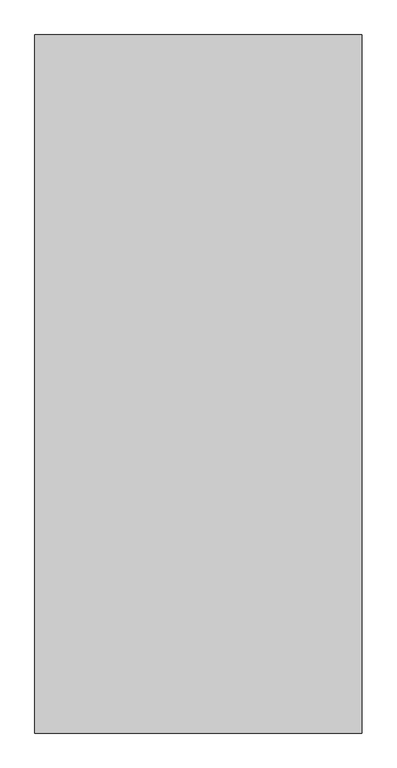
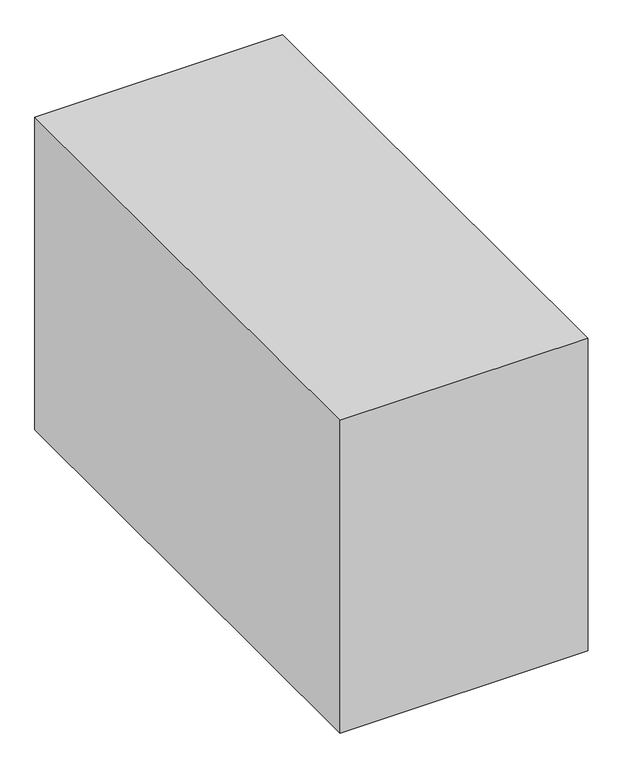
"""IFC4 building model written with IfcOpenShell, lengths in millimetres: proxy geometry, Space Planning Box_hec : Space Planning Box_hec."""

import ifcopenshell
import ifcopenshell.guid

model = None  # the IFC model being written
_history = None  # IfcOwnerHistory: only IFC2X3 demands one
_inside = {}  # id of a spatial element -> (the spatial element, [elements in it])
_under = {}  # id of a project, library or spatial element -> (it, [spatial elements below it])
_declared = {}  # id of a project -> (the project, [libraries it declares])
_typed = {}  # id of a type object -> (the type object, [elements of that type])
_made_of = {}  # id of a material, layer set ... -> (it, [elements and type objects made of it])


def new_model(schema):
    """Start an empty IFC model of exactly this schema.

    Asked for "IFC4X3", IfcOpenShell would pick the latest addendum, in which some entities
    have other attributes; the version numbers below select the first issue.
    IFC2X3 requires an IfcOwnerHistory on every rooted entity: one is made here for all.
    """
    global model, _history
    if schema == "IFC4X3":
        model = ifcopenshell.file(schema_version=(4, 3, 0, 0))
    else:
        model = ifcopenshell.file(schema=schema)
    _inside.clear()
    _under.clear()
    _declared.clear()
    _typed.clear()
    _made_of.clear()
    _history = None
    if model.schema == "IFC2X3":
        org = make("IfcOrganization", Name="unknown")
        user = make(
            "IfcPersonAndOrganization",
            ThePerson=make("IfcPerson", FamilyName="unknown"),
            TheOrganization=org,
        )
        app = make(
            "IfcApplication",
            ApplicationDeveloper=org,
            Version="unknown",
            ApplicationFullName="unknown",
            ApplicationIdentifier="unknown",
        )
        _history = make(
            "IfcOwnerHistory",
            OwningUser=user,
            OwningApplication=app,
            ChangeAction="ADDED",
            CreationDate=0,
        )
    return model


def make(cls, **values):
    """One entity of the class cls with the attributes given. An attribute that is None is left unset."""
    return model.create_entity(
        cls, **{name: value for name, value in values.items() if value is not None}
    )


def rooted(cls, **values):
    """An entity with a GlobalId (a new one), such as an element, a storey or a relation."""
    return make(cls, GlobalId=ifcopenshell.guid.new(), OwnerHistory=_history, **values)


def si_unit(unit_type, name, prefix=None):
    """IfcSIUnit, for example si_unit("LENGTHUNIT", "METRE", prefix="MILLI")."""
    return make("IfcSIUnit", UnitType=unit_type, Prefix=prefix, Name=name)


def assignment(units):
    """IfcUnitAssignment: the units of a project."""
    return None if units is None else make("IfcUnitAssignment", Units=units)


def point(xyz):
    """IfcCartesianPoint."""
    return None if xyz is None else make("IfcCartesianPoint", Coordinates=xyz)


def direction(xyz):
    """IfcDirection."""
    return None if xyz is None else make("IfcDirection", DirectionRatios=xyz)


def frame(location, z_axis=None, x_axis=None):
    """IfcAxis2Placement3D, a coordinate frame: its origin and axes. An axis left out is left unset."""
    return make(
        "IfcAxis2Placement3D",
        Location=point(location),
        Axis=direction(z_axis),
        RefDirection=direction(x_axis),
    )


def origin():
    """The frame at (0, 0, 0) with its axes left unset."""
    return frame((0.0, 0.0, 0.0))


def origin_with_axes():
    """The frame at (0, 0, 0) with the z axis (0, 0, 1) and the x axis (1, 0, 0) written out."""
    return frame((0.0, 0.0, 0.0), z_axis=(0.0, 0.0, 1.0), x_axis=(1.0, 0.0, 0.0))


def place(relative_to, where):
    """IfcLocalPlacement: puts the frame where relative to a parent placement (None: the world)."""
    return make(
        "IfcLocalPlacement", PlacementRelTo=relative_to, RelativePlacement=where
    )


def context(
    kind, dimensions, precision=None, world=None, true_north=None, identifier=None
):
    """IfcGeometricRepresentationContext, for example the 3D "Model" context."""
    return make(
        "IfcGeometricRepresentationContext",
        ContextIdentifier=identifier,
        ContextType=kind,
        CoordinateSpaceDimension=dimensions,
        Precision=precision,
        WorldCoordinateSystem=world,
        TrueNorth=true_north,
    )


def project(units=None, contexts=None):
    """IfcProject with its units and contexts."""
    return rooted(
        "IfcProject",
        Name="project",
        RepresentationContexts=contexts,
        UnitsInContext=assignment(units),
    )


def spatial(cls, under=None, at=None, **own):
    """A site, building, storey or space (cls), placed at a placement, below another one or the project."""
    s = rooted(cls, ObjectPlacement=at, **own)
    if under is not None:
        _under.setdefault(under.id(), (under, []))[1].append(s)
    return s


def polyline(points):
    """IfcPolyline through the points."""
    return make("IfcPolyline", Points=[point(p) for p in points])


def outline(outer, holes=None, kind="AREA"):
    """IfcArbitraryClosedProfileDef: a profile drawn as a closed curve; with holes, ...WithVoids."""
    if holes is None:
        return make("IfcArbitraryClosedProfileDef", ProfileType=kind, OuterCurve=outer)
    return make(
        "IfcArbitraryProfileDefWithVoids",
        ProfileType=kind,
        OuterCurve=outer,
        InnerCurves=holes,
    )


def extrude(swept, where, along, depth):
    """IfcExtrudedAreaSolid: the profile swept, set in the frame where, extruded along a direction by depth."""
    return make(
        "IfcExtrudedAreaSolid",
        SweptArea=swept,
        Position=where,
        ExtrudedDirection=direction(along),
        Depth=depth,
    )


def shape(context_of_items, identifier, shape_type, items):
    """IfcShapeRepresentation: the items that make up one representation, for example the "Body"."""
    return make(
        "IfcShapeRepresentation",
        ContextOfItems=context_of_items,
        RepresentationIdentifier=identifier,
        RepresentationType=shape_type,
        Items=items,
    )


def source(mapping_origin, context_of_items, identifier, shape_type, items):
    """IfcRepresentationMap: a shape defined once, which mapped items show again and again."""
    return make(
        "IfcRepresentationMap",
        MappingOrigin=mapping_origin,
        MappedRepresentation=shape(context_of_items, identifier, shape_type, items),
    )


def transform(
    local_origin,
    x_axis=None,
    y_axis=None,
    z_axis=None,
    scale=None,
    scale2=None,
    scale3=None,
    uniform=True,
):
    """IfcCartesianTransformationOperator3D, or its non-uniform kind. x_axis, y_axis, z_axis: its Axis1, 2, 3."""
    if uniform:
        return make(
            "IfcCartesianTransformationOperator3D",
            Axis1=direction(x_axis),
            Axis2=direction(y_axis),
            LocalOrigin=point(local_origin),
            Scale=scale,
            Axis3=direction(z_axis),
        )
    return make(
        "IfcCartesianTransformationOperator3DnonUniform",
        Axis1=direction(x_axis),
        Axis2=direction(y_axis),
        LocalOrigin=point(local_origin),
        Scale=scale,
        Axis3=direction(z_axis),
        Scale2=scale2,
        Scale3=scale3,
    )


def mapped(mapping_source, mapping_target):
    """IfcMappedItem: shows the shape of a source again, moved by a transform."""
    return make(
        "IfcMappedItem", MappingSource=mapping_source, MappingTarget=mapping_target
    )


def made_of(thing, what):
    """Note that an element or type object is made of a material, layer set ...; save() writes the relation."""
    if what is not None:
        _made_of.setdefault(what.id(), (what, []))[1].append(thing)
    return thing


def element(
    cls,
    number,
    at=None,
    inside=None,
    cuts=None,
    type_object=None,
    material=None,
    context=None,
    identifier="Body",
    shape_type=None,
    held_by="IfcProductDefinitionShape",
    body=None,
    shapes=None,
    **own,
):
    """One element of the class cls, such as IfcWall. Its Tag is "e" and its number.

    at: its placement. inside: the storey or other place that contains it. cuts: it is an
    opening in that element (IfcRelVoidsElement). A single representation is given by context,
    identifier, shape_type and body (its items); several are given by shapes. held_by: the class
    of the entity that holds the representations. save() writes the other relations.
    """
    e = rooted(cls, Tag="e%d" % number, ObjectPlacement=at, **own)
    if body is not None:
        shapes = [shape(context, identifier, shape_type, body)]
    if shapes is not None:
        e.Representation = make(held_by, Representations=shapes)
    if inside is not None:
        _inside.setdefault(inside.id(), (inside, []))[1].append(e)
    if cuts is not None:
        rooted(
            "IfcRelVoidsElement", RelatingBuildingElement=cuts, RelatedOpeningElement=e
        )
    if type_object is not None:
        _typed.setdefault(type_object.id(), (type_object, []))[1].append(e)
    return made_of(e, material)


def aggregate(whole, parts):
    """IfcRelAggregates: a whole, such as a stair, and the parts it consists of."""
    return rooted("IfcRelAggregates", RelatingObject=whole, RelatedObjects=parts)


def save(model, path):
    """Write the relations noted so far, then the file.

    IfcRelAggregates (storeys below a building ...), IfcRelContainedInSpatialStructure (elements
    in a storey), IfcRelDefinesByType, IfcRelAssociatesMaterial and IfcRelDeclares: one each for
    every whole, place, type object, material and project.
    """
    for whole, parts in _under.values():
        aggregate(whole, parts)
    for where, things in _inside.values():
        rooted(
            "IfcRelContainedInSpatialStructure",
            RelatedElements=things,
            RelatingStructure=where,
        )
    for kind, things in _typed.values():
        rooted("IfcRelDefinesByType", RelatedObjects=things, RelatingType=kind)
    for what, things in _made_of.values():
        rooted("IfcRelAssociatesMaterial", RelatedObjects=things, RelatingMaterial=what)
    for by, libraries in _declared.values():
        rooted("IfcRelDeclares", RelatingContext=by, RelatedDefinitions=libraries)
    model.write(path)


def generic_models_96097b63(model_context):
    return source(origin(), model_context, "Body", "SweptSolid", [
        extrude(outline(polyline([(2250.0, 4800.0), (2250.0, -4800.0), (-2250.0, -4800.0), (-2250.0, 4800.0), (2250.0, 4800.0)])), origin_with_axes(), (0.0, 0.0, 1.0), 6000.0),
    ])


if __name__ == "__main__":
    model = new_model("IFC4")
    model_context = context("Model", 3, world=origin())
    ifc_project = project(units=[si_unit("LENGTHUNIT", "METRE", prefix="MILLI")], contexts=[model_context])
    site = spatial("IfcSite", under=ifc_project)
    building = spatial("IfcBuilding", under=site)
    placement = place(None, origin())
    generic_models_shape = generic_models_96097b63(model_context)
    element("IfcBuildingElementProxy", 1, Name="Space Planning Box_hec : Space Planning Box_hec", ObjectType="Space Planning Box_hec : Space Planning Box_hec", at=placement, inside=building, context=model_context, shape_type="MappedRepresentation", body=[
        mapped(generic_models_shape, transform((0.0, 0.0, 0.0), x_axis=(1.0, 0.0, 0.0), y_axis=(0.0, 1.0, 0.0), z_axis=(0.0, 0.0, 1.0))),
    ])
    save(model, "model.ifc")

# Revit data of these elements
# Type "Space Planning Box_hec : Space Planning Box_hec"
#   Type Comments = "..."
#   Room Name [instance default] = "?"
#   Interior Finish [instance default] = ""
#   Exterior Finish [instance default] = ""
#   Department [instance default] = ""
#   Assembly Code = "..."
#   Width [instance default] = 1524 mm
#   Program Area [instance default] = 0.00 m²
#   Length [instance default] = 1524 mm
#   Height [instance default] = 1524 mm
#   Area [instance default] = 2.32258 m²
#   Fill Color [instance default] = Cyan
#   Default Elevation = 0
# Element 1 (IfcBuildingElementProxy, "Space Planning Box_hec : Space Planning Box_hec")
#   Room Name = "Shift Office Room"
#   Interior Finish = "IF2-1"
#   Exterior Finish = "EF1"
#   Department = "AR"
#   Width = 4500 mm
#   Program Area = 43.20 m²
#   Length = 9600 mm
#   Height = 6000 mm
#   Area = 43.20 m²
#   Materials on its faces: "Cyan"
# Materials
#   "Cyan": class "Generic", colour RGB 0 255 255, transparency 0.2, Cost = 0
